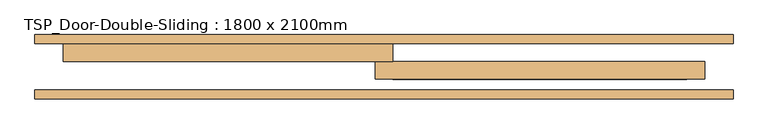
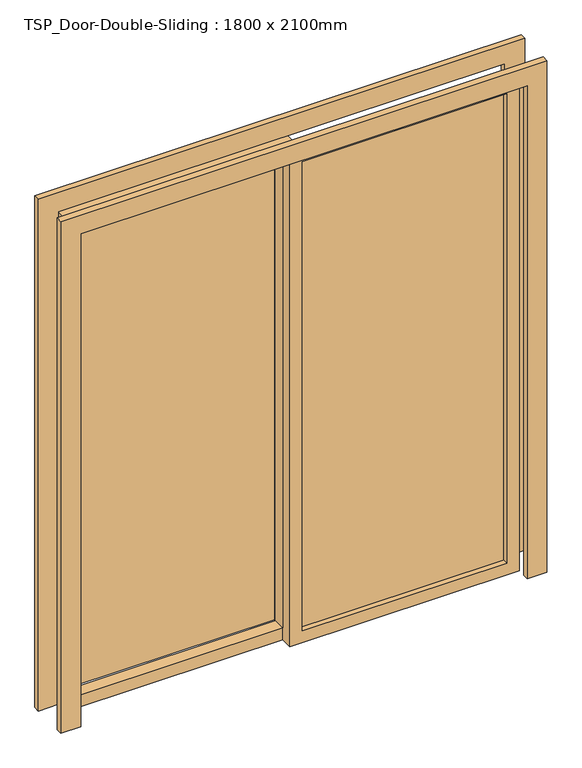
"""IFC4 building model written with IfcOpenShell, lengths in millimetres: door geometry, TSP_Door-Double-Sliding : 1800 x 2100mm."""

from ifc_helpers import new_model, si_unit, frame, origin, place, context, project, spatial, polyline, outline, extrude, source, transform, mapped, element, save


def tsp_door_double_sliding_1800_x_2100mm_68247d87(model_context):
    return source(origin(), model_context, "Body", "SweptSolid", [
        extrude(outline(polyline([(0.0, 980.0), (2180.0, 980.0), (2180.0, -980.0), (0.0, -980.0), (0.0, -900.0), (2100.0, -900.0), (2100.0, 900.0), (0.0, 900.0), (0.0, 980.0)])), frame((0.0, 192.0, 0.0), z_axis=(0.0, 1.0, 0.0), x_axis=(0.0, 0.0, 1.0)), (0.0, 0.0, 1.0), 25.0),
        extrude(outline(polyline([(0.0, -980.0), (0.0, -900.0), (2100.0, -900.0), (2100.0, 900.0), (0.0, 900.0), (0.0, 980.0), (2180.0, 980.0), (2180.0, -980.0), (0.0, -980.0)])), frame((0.0, 37.0, 0.0), z_axis=(0.0, 1.0, 0.0), x_axis=(0.0, 0.0, 1.0)), (0.0, 0.0, 1.0), 25.0),
        extrude(outline(polyline([(2100.0, 25.0), (2100.0, -900.0), (0.0, -900.0), (0.0, 25.0), (2100.0, 25.0)]), holes=[polyline([(2050.0, -25.0), (50.0, -25.0), (50.0, -850.0), (2050.0, -850.0), (2050.0, -25.0)])]), frame((0.0, 142.0, 0.0), z_axis=(0.0, 1.0, 0.0), x_axis=(0.0, 0.0, 1.0)), (0.0, 0.0, 1.0), 50.0),
        extrude(outline(polyline([(2100.0, -25.0), (0.0, -25.0), (0.0, 900.0), (2100.0, 900.0), (2100.0, -25.0)]), holes=[polyline([(2050.0, 25.0), (2050.0, 850.0), (50.0, 850.0), (50.0, 25.0), (2050.0, 25.0)])]), frame((0.0, 92.0, 0.0), z_axis=(0.0, 1.0, 0.0), x_axis=(0.0, 0.0, 1.0)), (0.0, 0.0, 1.0), 50.0),
        extrude(outline(polyline([(-25.0, 200.025), (-850.0, 200.025), (-850.0, 206.375), (-25.0, 206.375), (-25.0, 200.025)])), frame((0.0, 0.0, 50.0), z_axis=(0.0, 0.0, 1.0), x_axis=(1.0, 0.0, 0.0)), (0.0, 0.0, 1.0), 2000.0),
        extrude(outline(polyline([(25.0, 120.175), (850.0, 120.175), (850.0, 113.825), (25.0, 113.825), (25.0, 120.175)])), frame((0.0, 0.0, 50.0), z_axis=(0.0, 0.0, 1.0), x_axis=(1.0, 0.0, 0.0)), (0.0, 0.0, 1.0), 2000.0),
    ])


if __name__ == "__main__":
    model = new_model("IFC4")
    model_context = context("Model", 3, world=origin())
    ifc_project = project(units=[si_unit("LENGTHUNIT", "METRE", prefix="MILLI")], contexts=[model_context])
    site = spatial("IfcSite", under=ifc_project)
    building = spatial("IfcBuilding", under=site)
    placement = place(None, origin())
    tsp_door_double_sliding_1800_x_2100mm_shape = tsp_door_double_sliding_1800_x_2100mm_68247d87(model_context)
    element("IfcDoor", 1, ObjectType="TSP_Door-Double-Sliding : 1800 x 2100mm", at=placement, inside=building, context=model_context, shape_type="MappedRepresentation", body=[
        mapped(tsp_door_double_sliding_1800_x_2100mm_shape, transform((0.0, 0.0, 0.0), x_axis=(1.0, 0.0, 0.0), y_axis=(0.0, 1.0, 0.0), z_axis=(0.0, 0.0, 1.0))),
    ])
    save(model, "model.ifc")

# Revit data of these elements
# Type "TSP_Door-Double-Sliding : 1800 x 2100mm"
#   Model = "TSP_DOOR01A"
#   Type Mark = "90"
#   Construction Type Id = "opn-d45"
#   Assembly Code = "C1020"
#   Analytic Construction = "Wood frame, double glass door "
#   Thickness = 50 mm
#   Thermal Resistance (R) = 0.31964 (m²·K)/W
#   Heat Transfer Coefficient (U) = 3.12872 W/(m²·K)
#   Height = 2100 mm
#   Rail Width = 50 mm
#   Stiles = 50 mm
#   Trim Projection Ext = 25 mm
#   Trim Projection Int = 25 mm
#   Trim Width = 80 mm
#   Width = 1800 mm
#   Define Thermal Properties by = 1
#   Glazing = Glass
#   Panel Material = Wood - Birch - Solid Stained Light Low Gloss
#   Trim Material = Paint - Sienna
#   Visual Light Transmittance = 0
#   Solar Heat Gain Coefficient = 0
#   Function = (empty or 0)
#   Wall Closure = (empty or 0)
# Element 1 (IfcDoor, "TSP_Door-Double-Sliding : 1800 x 2100mm")
#   Materials on its faces: "Paint - Sienna", "Wood - Birch - Solid Stained Light Low Gloss", "Glass"
# Materials
#   "Glass": class "Glass", colour RGB 0 128 192, transparency 0.9, Description = "Soda Lime Glass", Cost = 0
#   "Wood - Birch - Solid Stained Light Low Gloss": class "Wood", colour RGB 210 159 95, transparency 0, Cost = 0
#   "Paint - Sienna": class "Miscellaneous", colour RGB 118 70 51, transparency 0, Cost = 0
